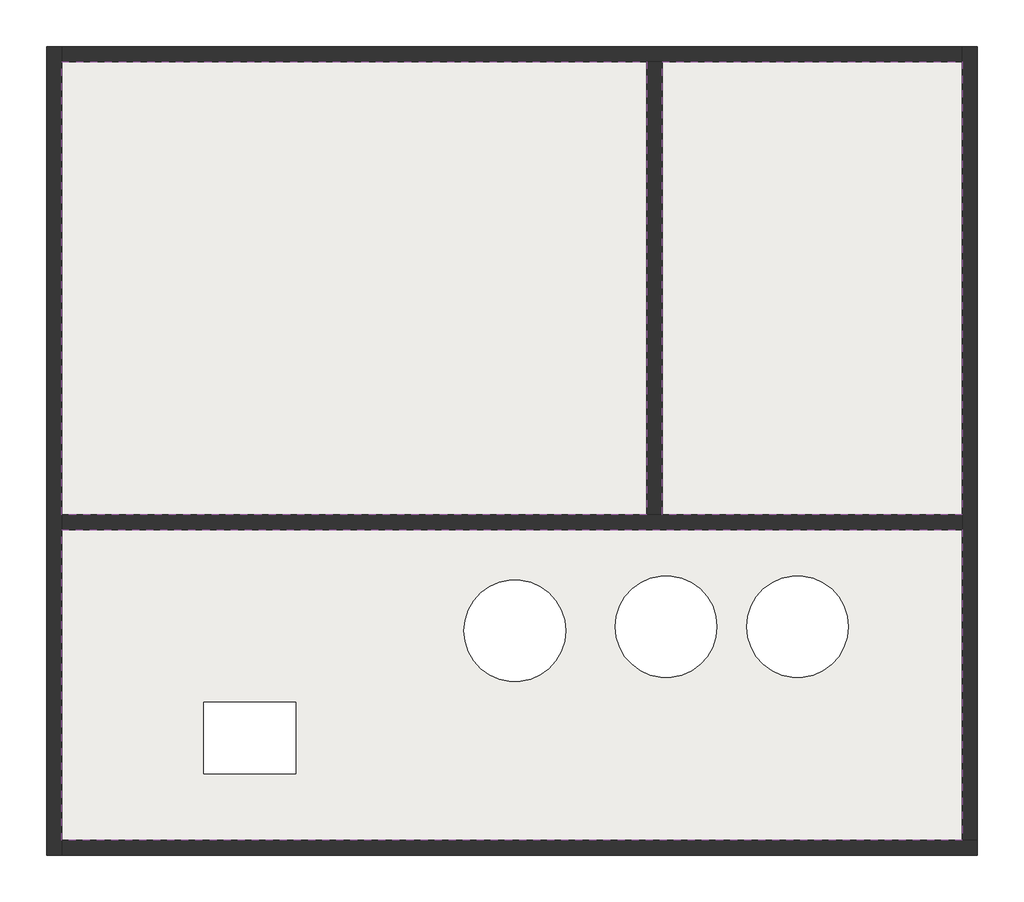
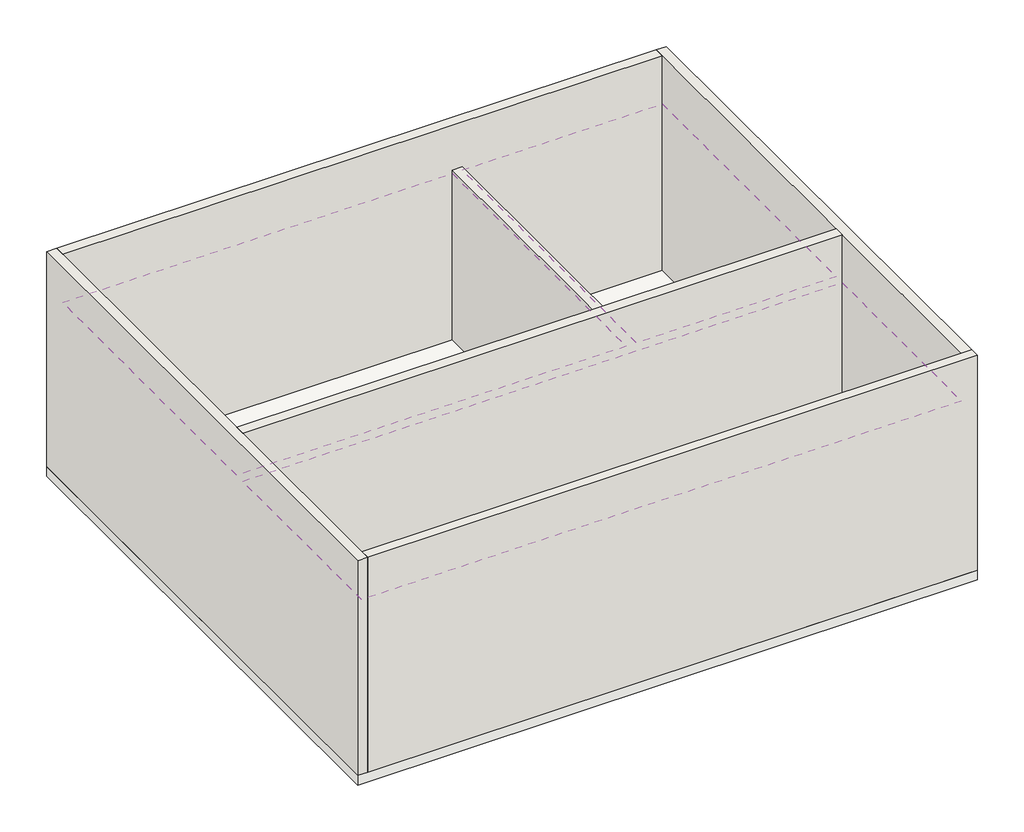
# One storey: 6 walls, 3 coverings, 1 slab.
"""IFC4 building model written with IfcOpenShell, lengths in millimetres."""

from ifc_helpers import new_model, si_unit, point, frame, frame_2d, origin, place, context, project, spatial, polyline, circle_curve, trimmed, segment, composite_curve, outline, extrude, faceted_brep, element, save

model = new_model("IFC4")

# Units and contexts
model_context = context("Model", 3, world=origin())
ifc_project = project(units=[si_unit("LENGTHUNIT", "METRE", prefix="MILLI")], contexts=[model_context])

# Site, building, storey
site = spatial("IfcSite", under=ifc_project)
building = spatial("IfcBuilding", under=site)
storey = spatial("IfcBuildingStorey", under=building, Name="レベル 1", Elevation=500.0)

# Coverings
placement = place(None, origin())
element("IfcCovering", 1, ObjectType="グリッド 600x600mm", at=placement, inside=storey, context=model_context, shape_type="SweptSolid", body=[
    extrude(outline(polyline([(-4139.1497645, -1548.6940898), (-9889.1497645, -1548.6940898), (-9889.1497645, 2901.3059102), (-4139.1497645, 2901.3059102), (-4139.1497645, -1548.6940898)])), frame((0.0, 0.0, 3100.0), z_axis=(0.0, 0.0, 1.0), x_axis=(1.0, 0.0, 0.0)), (0.0, 0.0, 1.0), 52.0),
])
element("IfcCovering", 2, ObjectType="グリッド 600x600mm", at=placement, inside=storey, context=model_context, shape_type="SweptSolid", body=[
    extrude(outline(polyline([(-1039.1497645, 2901.3059102), (-1039.1497645, -1548.6940898), (-3989.1497645, -1548.6940898), (-3989.1497645, 2901.3059102), (-1039.1497645, 2901.3059102)])), frame((0.0, 0.0, 3100.0), z_axis=(0.0, 0.0, 1.0), x_axis=(1.0, 0.0, 0.0)), (0.0, 0.0, 1.0), 52.0),
])
element("IfcCovering", 3, ObjectType="グリッド 600x600mm", at=placement, inside=storey, context=model_context, shape_type="SweptSolid", body=[
    extrude(outline(polyline([(-1039.1497645, -1698.6940898), (-1039.1497645, -4748.6940898), (-9889.1497645, -4748.6940898), (-9889.1497645, -1698.6940898), (-1039.1497645, -1698.6940898)]), holes=[polyline([(-7591.6429011, -4094.9873293), (-7591.6429011, -3394.9873293), (-8491.6429011, -3394.9873293), (-8491.6429011, -4094.9873293), (-7591.6429011, -4094.9873293)]), composite_curve([segment(trimmed(circle_curve(frame_2d((-5436.6640818, -2690.8635378)), 500.0), [point((-5436.6640818, -2190.8635378))], [point((-5436.6640818, -3190.8635378))], True, "CARTESIAN"), True, "CONTINUOUS"), segment(trimmed(circle_curve(frame_2d((-5436.6640818, -2690.8635378)), 500.0), [point((-5436.6640818, -3190.8635378))], [point((-5436.6640818, -2190.8635378))], True, "CARTESIAN"), True, "CONTINUOUS")], self_intersect=False), composite_curve([segment(trimmed(circle_curve(frame_2d((-3949.3788791, -2650.2471348)), 500.0), [point((-3949.3788791, -2150.2471348))], [point((-3949.3788791, -3150.2471348))], True, "CARTESIAN"), True, "CONTINUOUS"), segment(trimmed(circle_curve(frame_2d((-3949.3788791, -2650.2471348)), 500.0), [point((-3949.3788791, -3150.2471348))], [point((-3949.3788791, -2150.2471348))], True, "CARTESIAN"), True, "CONTINUOUS")], self_intersect=False), composite_curve([segment(trimmed(circle_curve(frame_2d((-2657.8130196, -2650.2471348)), 500.0), [point((-2657.8130196, -2150.2471348))], [point((-2657.8130196, -3150.2471348))], True, "CARTESIAN"), True, "CONTINUOUS"), segment(trimmed(circle_curve(frame_2d((-2657.8130196, -2650.2471348)), 500.0), [point((-2657.8130196, -3150.2471348))], [point((-2657.8130196, -2150.2471348))], True, "CARTESIAN"), True, "CONTINUOUS")], self_intersect=False)]), frame((0.0, 0.0, 3100.0), z_axis=(0.0, 0.0, 1.0), x_axis=(1.0, 0.0, 0.0)), (0.0, 0.0, 1.0), 52.0),
])

# Slab
element("IfcSlab", 4, ObjectType="一般 150 mm", at=placement, inside=storey, context=model_context, shape_type="SweptSolid", body=[
    extrude(outline(polyline([(-889.1497645, 3051.3059102), (-889.1497645, -4898.6940898), (-10039.1497645, -4898.6940898), (-10039.1497645, 3051.3059102), (-889.1497645, 3051.3059102)]), holes=[polyline([(-7591.6429011, -3394.9873293), (-8491.6429011, -3394.9873293), (-8491.6429011, -4094.9873293), (-7591.6429011, -4094.9873293), (-7591.6429011, -3394.9873293)]), composite_curve([segment(trimmed(circle_curve(frame_2d((-5436.6640818, -2690.8635378)), 500.0), [point((-4936.6640818, -2690.8635378))], [point((-5936.6640818, -2690.8635378))], True, "CARTESIAN"), True, "CONTINUOUS"), segment(trimmed(circle_curve(frame_2d((-5436.6640818, -2690.8635378)), 500.0), [point((-5936.6640818, -2690.8635378))], [point((-4936.6640818, -2690.8635378))], True, "CARTESIAN"), True, "CONTINUOUS")], self_intersect=False), composite_curve([segment(trimmed(circle_curve(frame_2d((-3949.3788791, -2650.2471348)), 500.0), [point((-3449.3788791, -2650.2471348))], [point((-4449.3788791, -2650.2471348))], True, "CARTESIAN"), True, "CONTINUOUS"), segment(trimmed(circle_curve(frame_2d((-3949.3788791, -2650.2471348)), 500.0), [point((-4449.3788791, -2650.2471348))], [point((-3449.3788791, -2650.2471348))], True, "CARTESIAN"), True, "CONTINUOUS")], self_intersect=False), composite_curve([segment(trimmed(circle_curve(frame_2d((-2657.8130196, -2650.2471348)), 500.0), [point((-2157.8130196, -2650.2471348))], [point((-3157.8130196, -2650.2471348))], True, "CARTESIAN"), True, "CONTINUOUS"), segment(trimmed(circle_curve(frame_2d((-2657.8130196, -2650.2471348)), 500.0), [point((-3157.8130196, -2650.2471348))], [point((-2157.8130196, -2650.2471348))], True, "CARTESIAN"), True, "CONTINUOUS")], self_intersect=False)]), frame((0.0, 0.0, 350.0), z_axis=(0.0, 0.0, 1.0), x_axis=(1.0, 0.0, 0.0)), (0.0, 0.0, 1.0), 150.0),
])

# Walls
element("IfcWall", 5, ObjectType="標準-150mm", at=placement, inside=storey, context=model_context, shape_type="Brep", body=[
    faceted_brep([(-10039.1497645, 3051.3059102, 500.0), (-10039.1497645, -4898.6940898, 500.0), (-10039.1497645, -4898.6940898, 3850.0), (-10039.1497645, 3051.3059102, 3850.0), (-9889.1497645, 3051.3059102, 500.0), (-9889.1497645, 3051.3059102, 3850.0), (-9889.1497645, 2901.3059102, 3850.0), (-9889.1497645, -1548.6940898, 3850.0), (-9889.1497645, -1698.6940898, 3850.0), (-9889.1497645, -4748.6940898, 3850.0), (-9889.1497645, -4898.6940898, 3850.0), (-9889.1497645, -4898.6940898, 500.0), (-9889.1497645, -4748.6940898, 500.0), (-9889.1497645, -1698.6940898, 500.0), (-9889.1497645, -1548.6940898, 500.0), (-9889.1497645, 2901.3059102, 500.0)], [[[0, 1, 2, 3]], [[4, 5, 6, 7, 8, 9, 10, 11, 12, 13, 14, 15]], [[1, 0, 4, 15, 14, 13, 12, 11]], [[3, 2, 10, 9, 8, 7, 6, 5]], [[0, 3, 5, 4]], [[2, 1, 11, 10]]]),
])
element("IfcWall", 6, ObjectType="標準-150mm", at=placement, inside=storey, context=model_context, shape_type="Brep", body=[
    faceted_brep([(-9889.1497645, -1698.6940898, 500.0), (-1039.1497645, -1698.6940898, 500.0), (-1039.1497645, -1698.6940898, 3850.0), (-9889.1497645, -1698.6940898, 3850.0), (-9889.1497645, -1548.6940898, 500.0), (-9889.1497645, -1548.6940898, 3850.0), (-1039.1497645, -1548.6940898, 3850.0), (-1039.1497645, -1548.6940898, 500.0), (-3989.1497645, -1548.6940898, 500.0), (-4139.1497645, -1548.6940898, 500.0)], [[[0, 1, 2, 3]], [[4, 5, 6, 7, 8, 9]], [[1, 0, 4, 9, 8, 7]], [[0, 3, 5, 4]], [[2, 1, 7, 6]], [[3, 2, 6, 5]]]),
])
element("IfcWall", 7, ObjectType="標準-150mm", at=placement, inside=storey, context=model_context, shape_type="Brep", body=[
    faceted_brep([(-889.1497645, -4748.6940898, 500.0), (-889.1497645, 3051.3059102, 500.0), (-889.1497645, 3051.3059102, 3850.0), (-889.1497645, -4748.6940898, 3850.0), (-1039.1497645, -4748.6940898, 500.0), (-1039.1497645, -4748.6940898, 3850.0), (-1039.1497645, -1698.6940898, 3850.0), (-1039.1497645, -1548.6940898, 3850.0), (-1039.1497645, 2901.3059102, 3850.0), (-1039.1497645, 3051.3059102, 3850.0), (-1039.1497645, 3051.3059102, 500.0), (-1039.1497645, 2901.3059102, 500.0), (-1039.1497645, -1548.6940898, 500.0), (-1039.1497645, -1698.6940898, 500.0)], [[[0, 1, 2, 3]], [[4, 5, 6, 7, 8, 9, 10, 11, 12, 13]], [[1, 0, 4, 13, 12, 11, 10]], [[3, 2, 9, 8, 7, 6, 5]], [[2, 1, 10, 9]], [[0, 3, 5, 4]]]),
])
element("IfcWall", 8, ObjectType="標準-150mm", at=placement, inside=storey, context=model_context, shape_type="Brep", body=[
    faceted_brep([(-1039.1497645, 3051.3059102, 500.0), (-9889.1497645, 3051.3059102, 500.0), (-9889.1497645, 3051.3059102, 3850.0), (-1039.1497645, 3051.3059102, 3850.0), (-1039.1497645, 2901.3059102, 500.0), (-1039.1497645, 2901.3059102, 3850.0), (-9889.1497645, 2901.3059102, 3850.0), (-9889.1497645, 2901.3059102, 500.0), (-4139.1497645, 2901.3059102, 500.0), (-3989.1497645, 2901.3059102, 500.0)], [[[0, 1, 2, 3]], [[4, 5, 6, 7, 8, 9]], [[1, 0, 4, 9, 8, 7]], [[3, 2, 6, 5]], [[2, 1, 7, 6]], [[0, 3, 5, 4]]]),
])
element("IfcWall", 9, ObjectType="標準-150mm", at=placement, inside=storey, context=model_context, shape_type="SweptSolid", body=[
    extrude(outline(polyline([(-4139.1497645, -1548.6940898), (-4139.1497645, 2901.3059102), (-3989.1497645, 2901.3059102), (-3989.1497645, -1548.6940898), (-4139.1497645, -1548.6940898)])), frame((0.0, 0.0, 500.0), z_axis=(0.0, 0.0, 1.0), x_axis=(1.0, 0.0, 0.0)), (0.0, 0.0, 1.0), 2652.0),
])
element("IfcWall", 10, ObjectType="標準-150mm", at=placement, inside=storey, context=model_context, shape_type="Brep", body=[
    faceted_brep([(-9889.1497645, -4898.6940898, 500.0), (-889.1497645, -4898.6940898, 500.0), (-889.1497645, -4898.6940898, 3850.0), (-9889.1497645, -4898.6940898, 3850.0), (-9889.1497645, -4748.6940898, 500.0), (-9889.1497645, -4748.6940898, 3850.0), (-1039.1497645, -4748.6940898, 3850.0), (-889.1497645, -4748.6940898, 3850.0), (-889.1497645, -4748.6940898, 500.0), (-1039.1497645, -4748.6940898, 500.0)], [[[0, 1, 2, 3]], [[4, 5, 6, 7, 8, 9]], [[1, 0, 4, 9, 8]], [[3, 2, 7, 6, 5]], [[0, 3, 5, 4]], [[2, 1, 8, 7]]]),
])

save(model, "model.ifc")

# Revit data of these elements
# Project information
#   プロジェクト発行日 = "発行日"
#   プロジェクト ステータス = "プロジェクト ステータス"
#   クライアント名 = "オーナ"
#   計画地住所 = "ここにアドレスを入力"
#   プロジェクト名 = "プロジェクト名"
#   プロジェクト番号 = "0001"
# Type "グリッド 600x600mm"
#   built-in parameter 1002203 = 1 (stored number, unit not read)
#   built-in parameter 1002202 = 1 (stored number, unit not read)
#   Layers, outside or top first: 36 mm no material (function 1); 16 mm "天井タイル 600 x 600" (function 5)
# Type "一般 150 mm"
#   Function = 0
#   Layers, outside or top first: 150 mm no material (function 1)
# Type "標準-150mm"
#   Layers, outside or top first: 150 mm no material (function 1)
# Elements 1, 2, 3 (IfcCovering, "グリッド 600x600mm")
#   Height Offset From Level = 2600 mm
#   Phase Created = 新しい建設
#   Materials on its faces: "天井タイル 600 x 600"
# Element 4 (IfcSlab, "一般 150 mm")
#   Height Offset From Level = 0 mm
#   Phase Created = 新しい建設
# Elements 5, 6, 7, 8, 10 (IfcWall, "標準-150mm")
#   Top Offset = 0 mm
#   Base Offset = 0 mm
#   wall height = 3350 mm
#   Phase Created = 新しい建設
#   Base Constraint = レベル 1
#   Top Constraint = レベル 2
#   Materials on its faces: "既定の壁"
# Element 9 (IfcWall, "標準-150mm")
#   Top Offset = -848 mm
#   Base Offset = 0 mm
#   wall height = 2652 mm
#   Phase Created = 新しい建設
#   Base Constraint = レベル 1
#   Top Constraint = レベル 2
#   Materials on its faces: "既定の壁"
# Materials
#   "天井タイル 600 x 600": class "一般", colour RGB 235 235 235, transparency 0, Description = "吸音天井タイル", Cost = 0
#   "既定の壁": class "その他", colour RGB 127 127 127, transparency 0, Cost = 0
